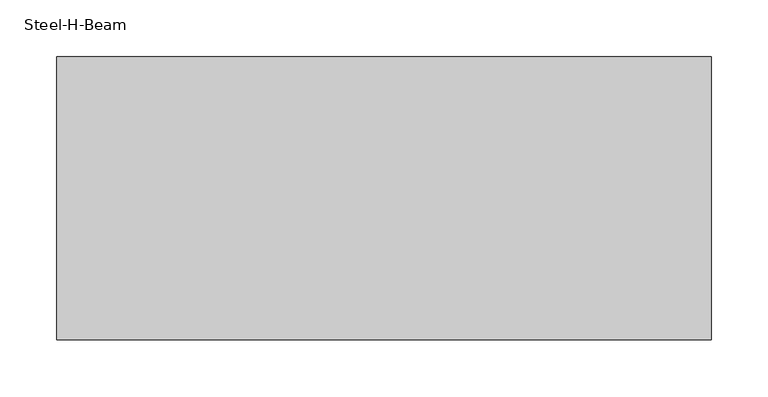
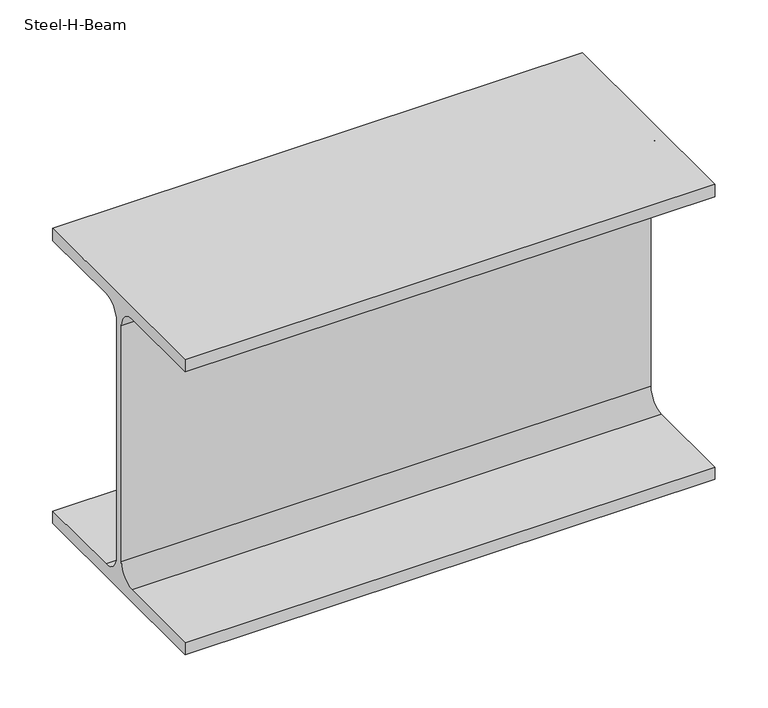
"""IFC4 building model written with IfcOpenShell, lengths in millimetres: beam geometry, Steel-H-Beam : BM121_H-340×250x9x14."""

from ifc_helpers import new_model, si_unit, point, frame, frame_2d, origin, place, context, project, spatial, polyline, circle_curve, trimmed, segment, composite_curve, outline, extrude, source, transform, mapped, element, save


def steel_h_beam_2abaa151(model_context):
    return source(origin(), model_context, "Body", "SweptSolid", [
        extrude(outline(composite_curve([segment(polyline([(-125.0, -156.0), (-24.5, -156.0)]), True, "CONTINUOUS"), segment(trimmed(circle_curve(frame_2d((-24.5, -136.0)), 20.0), [point((-24.5, -156.0))], [point((-4.5, -136.0))], True, "CARTESIAN"), True, "CONTINUOUS"), segment(polyline([(-4.5, -136.0), (-4.5, 136.0)]), True, "CONTINUOUS"), segment(trimmed(circle_curve(frame_2d((-24.5, 136.0)), 20.0), [point((-4.5, 136.0))], [point((-24.5, 156.0))], True, "CARTESIAN"), True, "CONTINUOUS"), segment(polyline([(-24.5, 156.0), (-125.0, 156.0), (-125.0, 170.0), (125.0, 170.0), (125.0, 156.0), (24.5, 156.0)]), True, "CONTINUOUS"), segment(trimmed(circle_curve(frame_2d((24.5, 136.0)), 20.0), [point((24.5, 156.0))], [point((4.5, 136.0))], True, "CARTESIAN"), True, "CONTINUOUS"), segment(polyline([(4.5, 136.0), (4.5, -136.0)]), True, "CONTINUOUS"), segment(trimmed(circle_curve(frame_2d((24.5, -136.0)), 20.0), [point((4.5, -136.0))], [point((24.5, -156.0))], True, "CARTESIAN"), True, "CONTINUOUS"), segment(polyline([(24.5, -156.0), (125.0, -156.0), (125.0, -170.0), (-125.0, -170.0), (-125.0, -156.0)]), True, "CONTINUOUS")], self_intersect=False)), frame((-362.6823513, 0.0, 0.0), z_axis=(1.0, 0.0, 0.0), x_axis=(0.0, 1.0, 0.0)), (0.0, 0.0, 1.0), 577.8891822),
    ])


if __name__ == "__main__":
    model = new_model("IFC4")
    model_context = context("Model", 3, world=origin())
    ifc_project = project(units=[si_unit("LENGTHUNIT", "METRE", prefix="MILLI")], contexts=[model_context])
    site = spatial("IfcSite", under=ifc_project)
    building = spatial("IfcBuilding", under=site)
    placement = place(None, origin())
    steel_h_beam_shape = steel_h_beam_2abaa151(model_context)
    element("IfcBeam", 1, ObjectType="Steel-H-Beam : BM121_H-340×250x9x14", at=placement, inside=building, context=model_context, shape_type="MappedRepresentation", body=[
        mapped(steel_h_beam_shape, transform((0.0, 0.0, 0.0), x_axis=(1.0, 0.0, 0.0), y_axis=(0.0, 1.0, 0.0), z_axis=(0.0, 0.0, 1.0))),
    ])
    save(model, "model.ifc")

# Revit data of these elements
# Type "Steel-H-Beam : BM121_H-340×250x9x14"
#   Surface Area = 1.62766 m²/m
#   Section Area = 101.514 cm²
#   Mass per Unit Length = 79.6882 kg/m
#   Length [instance default] = 3000 mm
#   B = 250 mm
#   H = 340 mm
#   r = 20 mm
#   tw = 9 mm
#   tf = 14 mm
#   hec_material4 [instance default] = none
#   hec_material3 [instance default] = none
#   hec_material2 [instance default] = none
#   hec_material1 [instance default] = none
#   Structural Material [instance default] = Steel, 45-345
#   Assembly Code = ""
# Element 1 (IfcBeam, "Steel-H-Beam : BM121_H-340×250x9x14")
#   hec_material3 = F01AC000-00002_Building/Shelter Fire Proofing Work_Intumescent Coating Type_1 hr. rating (UL 1709))
#   hec_material2 = S01AA010-00002_Main Steel Structure Fabrication Work_Shelter/Building_Steel Painting/Coating_for Fireproofed Steel Surface, Surface Preparation & Primer Coat
#   hec_material1 = S03AA028-00001_Main Steel Structure Erection Work_Shelter/Building_Medium Steel
#   Structural Material = S01AA002-00001_Main Steel Structure Fabrication Work_Shelter/Building_Medium Steel - Standard
#   Materials on its faces: "S01AA002-00001_Main Steel Structure Fabrication Work_Shelter/Building_Medium Steel - Standard"
# Materials
#   "Steel, 45-345": class "Metal", colour RGB 189 187 185, transparency 0, Description = "Steel 345 MPa", Cost = 0
#   "S01AA002-00001_Main Steel Structure Fabrication Work_Shelter/Building_Medium Steel - Standard": class "Metal", colour RGB 120 120 120, transparency 0, Comments = "(90KG/M>Weight≥30KG/M)", Description = "Structural steel 50ksi", W00) Work Master Code = "S01AA002-0001", W01) Work Master_Lv1 = "Main Steel Structure Fabrication Work", W02) Work Master_Lv2 = "Shelter/Building", W03) Work Master_Spec.1 = "Medium Steel - Standard (90KG/M>Weight≥30KG/M)", Cost = 0
#   "F01AC000-00002_Building/Shelter Fire Proofing Work_Intumescent Coating Type_1 hr. rating (UL 1709))": class "Metal", colour RGB 255 128 128, transparency 0, Description = "Paint finished steel", W00) Work Master Code = "F01AC000-00002", W01) Work Master_Lv1 = "Building/Shelter Fire Proofing Work", W02) Work Master_Lv2 = "Intumescent Coating Type", W03) Work Master_Spec.1 = "1 hr. rating (UL 1709)", Cost = 0
#   "S01AA010-00002_Main Steel Structure Fabrication Work_Shelter/Building_Steel Painting/Coating_for Fireproofed Steel Surface, Surface Preparation & Primer Coat": class "Metal", colour RGB 120 120 120, transparency 0, Description = "Paint finished steel", W00) Work Master Code = "SS01AA010-00002", W01) Work Master_Lv1 = "Main Steel Structure Fabrication Work", W02) Work Master_Lv2 = "Shelter/Building", W03) Work Master_Spec.1 = "Steel Painting/Coating", W04) Work Master_Spec.2 = "for Fireproofed Steel Surface, Surface Preparation & Primer Coat", Cost = 0
#   "S03AA028-00001_Main Steel Structure Erection Work_Shelter/Building_Medium Steel": class "Metal", colour RGB 120 120 120, transparency 0, Comments = "(90KG/M>Weight≥30KG/M)", Description = "Structural steel 50ksi", W00) Work Master Code = "S03AA028-0001", W01) Work Master_Lv1 = "Main Steel Structure Erection Work", W02) Work Master_Lv2 = "Shelter/Building", W03) Work Master_Spec.1 = "Medium Steel (90KG/M>Weight≥30KG/M)", Cost = 0
